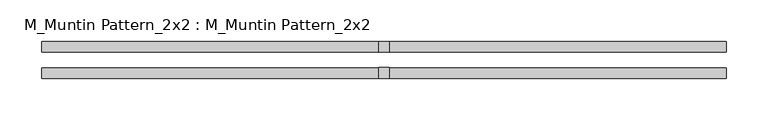
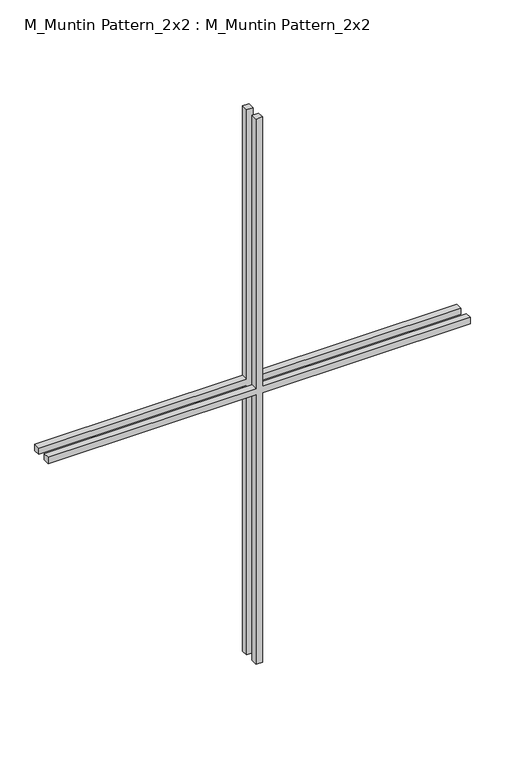
"""IFC4 building model written with IfcOpenShell, lengths in millimetres: proxy geometry, M_Muntin Pattern_2x2 : M_Muntin Pattern_2x2."""

import ifcopenshell
import ifcopenshell.guid

model = None  # the IFC model being written
_history = None  # IfcOwnerHistory: only IFC2X3 demands one
_inside = {}  # id of a spatial element -> (the spatial element, [elements in it])
_under = {}  # id of a project, library or spatial element -> (it, [spatial elements below it])
_declared = {}  # id of a project -> (the project, [libraries it declares])
_typed = {}  # id of a type object -> (the type object, [elements of that type])
_made_of = {}  # id of a material, layer set ... -> (it, [elements and type objects made of it])


def new_model(schema):
    """Start an empty IFC model of exactly this schema.

    Asked for "IFC4X3", IfcOpenShell would pick the latest addendum, in which some entities
    have other attributes; the version numbers below select the first issue.
    IFC2X3 requires an IfcOwnerHistory on every rooted entity: one is made here for all.
    """
    global model, _history
    if schema == "IFC4X3":
        model = ifcopenshell.file(schema_version=(4, 3, 0, 0))
    else:
        model = ifcopenshell.file(schema=schema)
    _inside.clear()
    _under.clear()
    _declared.clear()
    _typed.clear()
    _made_of.clear()
    _history = None
    if model.schema == "IFC2X3":
        org = make("IfcOrganization", Name="unknown")
        user = make(
            "IfcPersonAndOrganization",
            ThePerson=make("IfcPerson", FamilyName="unknown"),
            TheOrganization=org,
        )
        app = make(
            "IfcApplication",
            ApplicationDeveloper=org,
            Version="unknown",
            ApplicationFullName="unknown",
            ApplicationIdentifier="unknown",
        )
        _history = make(
            "IfcOwnerHistory",
            OwningUser=user,
            OwningApplication=app,
            ChangeAction="ADDED",
            CreationDate=0,
        )
    return model


def make(cls, **values):
    """One entity of the class cls with the attributes given. An attribute that is None is left unset."""
    return model.create_entity(
        cls, **{name: value for name, value in values.items() if value is not None}
    )


def rooted(cls, **values):
    """An entity with a GlobalId (a new one), such as an element, a storey or a relation."""
    return make(cls, GlobalId=ifcopenshell.guid.new(), OwnerHistory=_history, **values)


def si_unit(unit_type, name, prefix=None):
    """IfcSIUnit, for example si_unit("LENGTHUNIT", "METRE", prefix="MILLI")."""
    return make("IfcSIUnit", UnitType=unit_type, Prefix=prefix, Name=name)


def assignment(units):
    """IfcUnitAssignment: the units of a project."""
    return None if units is None else make("IfcUnitAssignment", Units=units)


def point(xyz):
    """IfcCartesianPoint."""
    return None if xyz is None else make("IfcCartesianPoint", Coordinates=xyz)


def direction(xyz):
    """IfcDirection."""
    return None if xyz is None else make("IfcDirection", DirectionRatios=xyz)


def frame(location, z_axis=None, x_axis=None):
    """IfcAxis2Placement3D, a coordinate frame: its origin and axes. An axis left out is left unset."""
    return make(
        "IfcAxis2Placement3D",
        Location=point(location),
        Axis=direction(z_axis),
        RefDirection=direction(x_axis),
    )


def origin():
    """The frame at (0, 0, 0) with its axes left unset."""
    return frame((0.0, 0.0, 0.0))


def place(relative_to, where):
    """IfcLocalPlacement: puts the frame where relative to a parent placement (None: the world)."""
    return make(
        "IfcLocalPlacement", PlacementRelTo=relative_to, RelativePlacement=where
    )


def context(
    kind, dimensions, precision=None, world=None, true_north=None, identifier=None
):
    """IfcGeometricRepresentationContext, for example the 3D "Model" context."""
    return make(
        "IfcGeometricRepresentationContext",
        ContextIdentifier=identifier,
        ContextType=kind,
        CoordinateSpaceDimension=dimensions,
        Precision=precision,
        WorldCoordinateSystem=world,
        TrueNorth=true_north,
    )


def project(units=None, contexts=None):
    """IfcProject with its units and contexts."""
    return rooted(
        "IfcProject",
        Name="project",
        RepresentationContexts=contexts,
        UnitsInContext=assignment(units),
    )


def spatial(cls, under=None, at=None, **own):
    """A site, building, storey or space (cls), placed at a placement, below another one or the project."""
    s = rooted(cls, ObjectPlacement=at, **own)
    if under is not None:
        _under.setdefault(under.id(), (under, []))[1].append(s)
    return s


def polyline(points):
    """IfcPolyline through the points."""
    return make("IfcPolyline", Points=[point(p) for p in points])


def outline(outer, holes=None, kind="AREA"):
    """IfcArbitraryClosedProfileDef: a profile drawn as a closed curve; with holes, ...WithVoids."""
    if holes is None:
        return make("IfcArbitraryClosedProfileDef", ProfileType=kind, OuterCurve=outer)
    return make(
        "IfcArbitraryProfileDefWithVoids",
        ProfileType=kind,
        OuterCurve=outer,
        InnerCurves=holes,
    )


def extrude(swept, where, along, depth):
    """IfcExtrudedAreaSolid: the profile swept, set in the frame where, extruded along a direction by depth."""
    return make(
        "IfcExtrudedAreaSolid",
        SweptArea=swept,
        Position=where,
        ExtrudedDirection=direction(along),
        Depth=depth,
    )


def shape(context_of_items, identifier, shape_type, items):
    """IfcShapeRepresentation: the items that make up one representation, for example the "Body"."""
    return make(
        "IfcShapeRepresentation",
        ContextOfItems=context_of_items,
        RepresentationIdentifier=identifier,
        RepresentationType=shape_type,
        Items=items,
    )


def source(mapping_origin, context_of_items, identifier, shape_type, items):
    """IfcRepresentationMap: a shape defined once, which mapped items show again and again."""
    return make(
        "IfcRepresentationMap",
        MappingOrigin=mapping_origin,
        MappedRepresentation=shape(context_of_items, identifier, shape_type, items),
    )


def transform(
    local_origin,
    x_axis=None,
    y_axis=None,
    z_axis=None,
    scale=None,
    scale2=None,
    scale3=None,
    uniform=True,
):
    """IfcCartesianTransformationOperator3D, or its non-uniform kind. x_axis, y_axis, z_axis: its Axis1, 2, 3."""
    if uniform:
        return make(
            "IfcCartesianTransformationOperator3D",
            Axis1=direction(x_axis),
            Axis2=direction(y_axis),
            LocalOrigin=point(local_origin),
            Scale=scale,
            Axis3=direction(z_axis),
        )
    return make(
        "IfcCartesianTransformationOperator3DnonUniform",
        Axis1=direction(x_axis),
        Axis2=direction(y_axis),
        LocalOrigin=point(local_origin),
        Scale=scale,
        Axis3=direction(z_axis),
        Scale2=scale2,
        Scale3=scale3,
    )


def mapped(mapping_source, mapping_target):
    """IfcMappedItem: shows the shape of a source again, moved by a transform."""
    return make(
        "IfcMappedItem", MappingSource=mapping_source, MappingTarget=mapping_target
    )


def made_of(thing, what):
    """Note that an element or type object is made of a material, layer set ...; save() writes the relation."""
    if what is not None:
        _made_of.setdefault(what.id(), (what, []))[1].append(thing)
    return thing


def element(
    cls,
    number,
    at=None,
    inside=None,
    cuts=None,
    type_object=None,
    material=None,
    context=None,
    identifier="Body",
    shape_type=None,
    held_by="IfcProductDefinitionShape",
    body=None,
    shapes=None,
    **own,
):
    """One element of the class cls, such as IfcWall. Its Tag is "e" and its number.

    at: its placement. inside: the storey or other place that contains it. cuts: it is an
    opening in that element (IfcRelVoidsElement). A single representation is given by context,
    identifier, shape_type and body (its items); several are given by shapes. held_by: the class
    of the entity that holds the representations. save() writes the other relations.
    """
    e = rooted(cls, Tag="e%d" % number, ObjectPlacement=at, **own)
    if body is not None:
        shapes = [shape(context, identifier, shape_type, body)]
    if shapes is not None:
        e.Representation = make(held_by, Representations=shapes)
    if inside is not None:
        _inside.setdefault(inside.id(), (inside, []))[1].append(e)
    if cuts is not None:
        rooted(
            "IfcRelVoidsElement", RelatingBuildingElement=cuts, RelatedOpeningElement=e
        )
    if type_object is not None:
        _typed.setdefault(type_object.id(), (type_object, []))[1].append(e)
    return made_of(e, material)


def aggregate(whole, parts):
    """IfcRelAggregates: a whole, such as a stair, and the parts it consists of."""
    return rooted("IfcRelAggregates", RelatingObject=whole, RelatedObjects=parts)


def save(model, path):
    """Write the relations noted so far, then the file.

    IfcRelAggregates (storeys below a building ...), IfcRelContainedInSpatialStructure (elements
    in a storey), IfcRelDefinesByType, IfcRelAssociatesMaterial and IfcRelDeclares: one each for
    every whole, place, type object, material and project.
    """
    for whole, parts in _under.values():
        aggregate(whole, parts)
    for where, things in _inside.values():
        rooted(
            "IfcRelContainedInSpatialStructure",
            RelatedElements=things,
            RelatingStructure=where,
        )
    for kind, things in _typed.values():
        rooted("IfcRelDefinesByType", RelatedObjects=things, RelatingType=kind)
    for what, things in _made_of.values():
        rooted("IfcRelAssociatesMaterial", RelatedObjects=things, RelatingMaterial=what)
    for by, libraries in _declared.values():
        rooted("IfcRelDeclares", RelatingContext=by, RelatedDefinitions=libraries)
    model.write(path)


def m_muntin_pattern_2x2_m_muntin_pattern_2x2_ad852c99(model_context):
    return source(origin(), model_context, "Body", "SweptSolid", [
        extrude(outline(polyline([(568.25, -6.35), (568.25, -411.9), (555.55, -411.9), (555.55, -6.35), (0.0, -6.35), (0.0, 6.35), (555.55, 6.35), (555.55, 411.9), (568.25, 411.9), (568.25, 6.35), (1123.8, 6.35), (1123.8, -6.35), (568.25, -6.35)])), frame((0.0, -22.225, 0.0), z_axis=(0.0, 1.0, 0.0), x_axis=(0.0, 0.0, 1.0)), (0.0, 0.0, 1.0), 12.7),
        extrude(outline(polyline([(568.25, -6.35), (568.25, -411.9), (555.55, -411.9), (555.55, -6.35), (0.0, -6.35), (0.0, 6.35), (555.55, 6.35), (555.55, 411.9), (568.25, 411.9), (568.25, 6.35), (1123.8, 6.35), (1123.8, -6.35), (568.25, -6.35)])), frame((0.0, 9.525, 0.0), z_axis=(0.0, 1.0, 0.0), x_axis=(0.0, 0.0, 1.0)), (0.0, 0.0, 1.0), 12.7),
    ])


if __name__ == "__main__":
    model = new_model("IFC4")
    model_context = context("Model", 3, world=origin())
    ifc_project = project(units=[si_unit("LENGTHUNIT", "METRE", prefix="MILLI")], contexts=[model_context])
    site = spatial("IfcSite", under=ifc_project)
    building = spatial("IfcBuilding", under=site)
    placement = place(None, origin())
    m_muntin_pattern_2x2_m_muntin_pattern_2x2_shape = m_muntin_pattern_2x2_m_muntin_pattern_2x2_ad852c99(model_context)
    element("IfcBuildingElementProxy", 1, Name="M_Muntin Pattern_2x2 : M_Muntin Pattern_2x2", ObjectType="M_Muntin Pattern_2x2 : M_Muntin Pattern_2x2", at=placement, inside=building, context=model_context, shape_type="MappedRepresentation", body=[
        mapped(m_muntin_pattern_2x2_m_muntin_pattern_2x2_shape, transform((0.0, 0.0, 0.0), x_axis=(1.0, 0.0, 0.0), y_axis=(0.0, 1.0, 0.0), z_axis=(0.0, 0.0, 1.0))),
    ])
    save(model, "model.ifc")

# Revit data of these elements
# Type "M_Muntin Pattern_2x2 : M_Muntin Pattern_2x2"
#   Width [instance default] = 1200 mm
#   Thickness = 12.7 mm
#   Height [instance default] = 1200 mm
#   Distance = 19.05 mm
#   Interior Material [instance default] = none
#   Exterior Material [instance default] = none
#   Default Elevation = 0
# Element 1 (IfcBuildingElementProxy, "M_Muntin Pattern_2x2 : M_Muntin Pattern_2x2")
#   Width = 823.8 mm
#   Height = 1123.8 mm
#   Interior Material = Wood - Stained
#   Exterior Material = Clad - White
#   Materials on its faces: "Clad - White", "Wood - Stained"
# Materials
#   "Clad - White": class "Wood", colour RGB 245 245 243, transparency 0, Cost = 0
#   "Wood - Stained": class "Wood", colour RGB 173 132 96, transparency 0, Cost = 0
